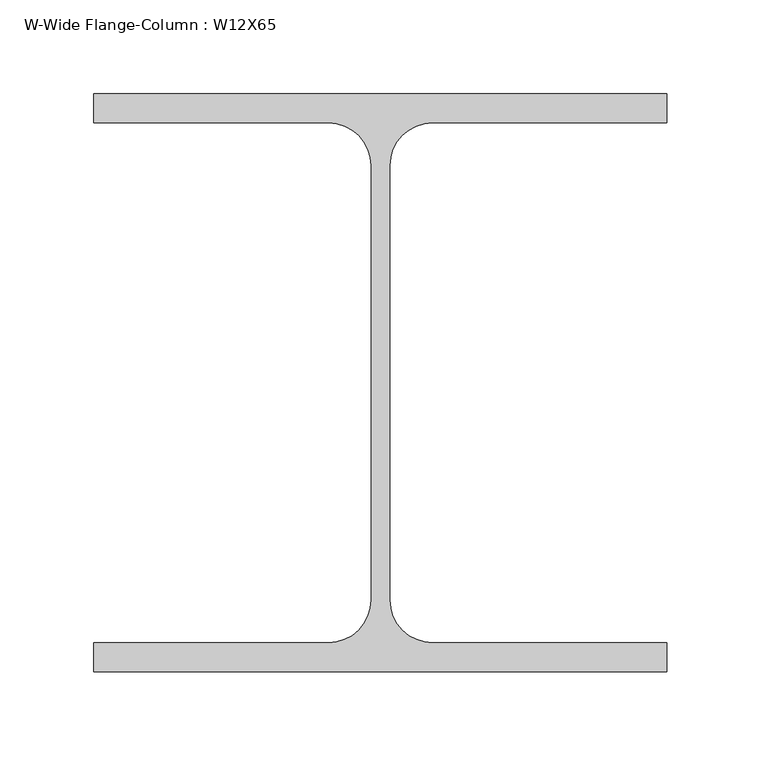
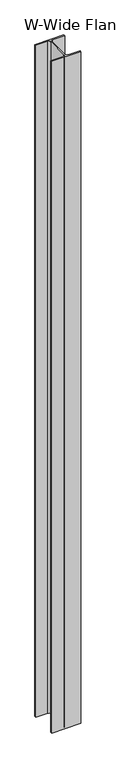
"""IFC4 building model written with IfcOpenShell, lengths in millimetres: column geometry, W-Wide Flange-Column : W12X65."""

from ifc_helpers import new_model, si_unit, point, frame, frame_2d, origin, place, context, project, spatial, polyline, circle_curve, trimmed, segment, composite_curve, outline, extrude, source, transform, mapped, element, save


def w_wide_flange_column_w12x65_6e4c071c(model_context):
    return source(origin(), model_context, "Body", "SweptSolid", [
        extrude(outline(composite_curve([segment(polyline([(152.4, 153.67), (152.4, 138.303), (27.686, 138.303)]), True, "CONTINUOUS"), segment(trimmed(circle_curve(frame_2d((27.686, 115.57)), 22.733), [point((27.686, 138.303))], [point((4.953, 115.57))], True, "CARTESIAN"), True, "CONTINUOUS"), segment(polyline([(4.953, 115.57), (4.953, -115.57)]), True, "CONTINUOUS"), segment(trimmed(circle_curve(frame_2d((27.686, -115.57)), 22.733), [point((4.953, -115.57))], [point((27.686, -138.303))], True, "CARTESIAN"), True, "CONTINUOUS"), segment(polyline([(27.686, -138.303), (152.4, -138.303), (152.4, -153.67), (-152.4, -153.67), (-152.4, -138.303), (-27.686, -138.303)]), True, "CONTINUOUS"), segment(trimmed(circle_curve(frame_2d((-27.686, -115.57)), 22.733), [point((-27.686, -138.303))], [point((-4.953, -115.57))], True, "CARTESIAN"), True, "CONTINUOUS"), segment(polyline([(-4.953, -115.57), (-4.953, 115.57)]), True, "CONTINUOUS"), segment(trimmed(circle_curve(frame_2d((-27.686, 115.57)), 22.733), [point((-4.953, 115.57))], [point((-27.686, 138.303))], True, "CARTESIAN"), True, "CONTINUOUS"), segment(polyline([(-27.686, 138.303), (-152.4, 138.303), (-152.4, 153.67), (152.4, 153.67)]), True, "CONTINUOUS")], self_intersect=False)), frame((0.0, 0.0, 8756.65), z_axis=(0.0, 0.0, 1.0), x_axis=(1.0, 0.0, 0.0)), (0.0, 0.0, 1.0), 7448.55),
    ])


if __name__ == "__main__":
    model = new_model("IFC4")
    model_context = context("Model", 3, world=origin())
    ifc_project = project(units=[si_unit("LENGTHUNIT", "METRE", prefix="MILLI")], contexts=[model_context])
    site = spatial("IfcSite", under=ifc_project)
    building = spatial("IfcBuilding", under=site)
    placement = place(None, origin())
    w_wide_flange_column_w12x65_shape = w_wide_flange_column_w12x65_6e4c071c(model_context)
    element("IfcColumn", 1, ObjectType="W-Wide Flange-Column : W12X65", at=placement, inside=building, context=model_context, shape_type="MappedRepresentation", body=[
        mapped(w_wide_flange_column_w12x65_shape, transform((0.0, 0.0, 0.0), x_axis=(1.0, 0.0, 0.0), y_axis=(0.0, 1.0, 0.0), z_axis=(0.0, 0.0, 1.0))),
    ])
    save(model, "model.ifc")

# Revit data of these elements
# Type "W-Wide Flange-Column : W12X65"
#   Assembly Code = "B10"
#   W = 65
#   bf = 1' - 0"
#   d = 1' - 0.1"
#   k = 0' - 1 1/2"
#   kr = 0' - 0.895"
#   tf = 0' - 0.605"
#   tw = 0' - 0.39"
#   A = 0.132639 SF
#   Structural Material [instance default] = Steel ASTM A992
# Element 1 (IfcColumn, "W-Wide Flange-Column : W12X65")
#   Materials on its faces: "Steel ASTM A992"
# Materials
#   "Steel ASTM A992": class "Metal", colour RGB 199 199 199, transparency 0, Description = "Structural steel 50ksi", Cost = 0
